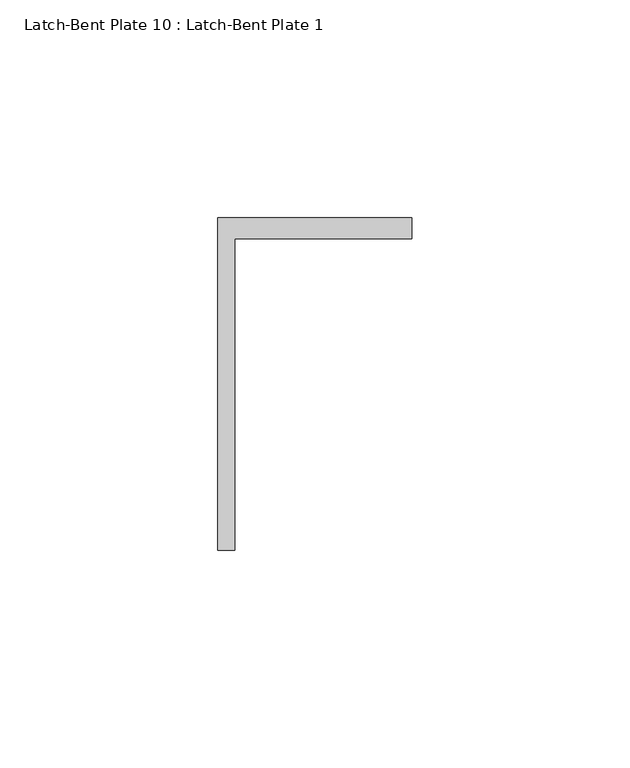
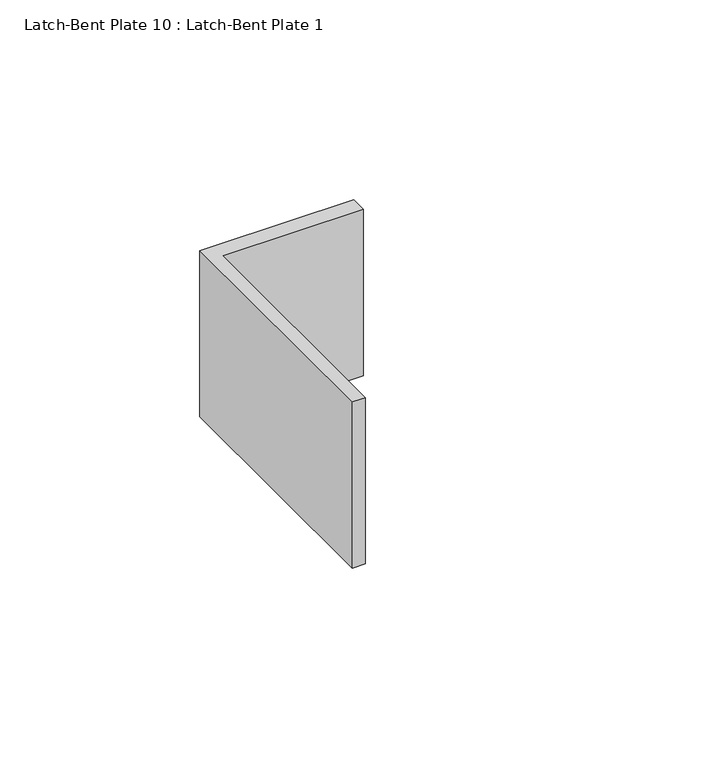
"""IFC4 building model written with IfcOpenShell, lengths in millimetres: proxy geometry, Latch-Bent Plate 10 : Latch-Bent Plate 1."""

import ifcopenshell
import ifcopenshell.guid

model = None  # the IFC model being written
_history = None  # IfcOwnerHistory: only IFC2X3 demands one
_inside = {}  # id of a spatial element -> (the spatial element, [elements in it])
_under = {}  # id of a project, library or spatial element -> (it, [spatial elements below it])
_declared = {}  # id of a project -> (the project, [libraries it declares])
_typed = {}  # id of a type object -> (the type object, [elements of that type])
_made_of = {}  # id of a material, layer set ... -> (it, [elements and type objects made of it])


def new_model(schema):
    """Start an empty IFC model of exactly this schema.

    Asked for "IFC4X3", IfcOpenShell would pick the latest addendum, in which some entities
    have other attributes; the version numbers below select the first issue.
    IFC2X3 requires an IfcOwnerHistory on every rooted entity: one is made here for all.
    """
    global model, _history
    if schema == "IFC4X3":
        model = ifcopenshell.file(schema_version=(4, 3, 0, 0))
    else:
        model = ifcopenshell.file(schema=schema)
    _inside.clear()
    _under.clear()
    _declared.clear()
    _typed.clear()
    _made_of.clear()
    _history = None
    if model.schema == "IFC2X3":
        org = make("IfcOrganization", Name="unknown")
        user = make(
            "IfcPersonAndOrganization",
            ThePerson=make("IfcPerson", FamilyName="unknown"),
            TheOrganization=org,
        )
        app = make(
            "IfcApplication",
            ApplicationDeveloper=org,
            Version="unknown",
            ApplicationFullName="unknown",
            ApplicationIdentifier="unknown",
        )
        _history = make(
            "IfcOwnerHistory",
            OwningUser=user,
            OwningApplication=app,
            ChangeAction="ADDED",
            CreationDate=0,
        )
    return model


def make(cls, **values):
    """One entity of the class cls with the attributes given. An attribute that is None is left unset."""
    return model.create_entity(
        cls, **{name: value for name, value in values.items() if value is not None}
    )


def rooted(cls, **values):
    """An entity with a GlobalId (a new one), such as an element, a storey or a relation."""
    return make(cls, GlobalId=ifcopenshell.guid.new(), OwnerHistory=_history, **values)


def si_unit(unit_type, name, prefix=None):
    """IfcSIUnit, for example si_unit("LENGTHUNIT", "METRE", prefix="MILLI")."""
    return make("IfcSIUnit", UnitType=unit_type, Prefix=prefix, Name=name)


def assignment(units):
    """IfcUnitAssignment: the units of a project."""
    return None if units is None else make("IfcUnitAssignment", Units=units)


def point(xyz):
    """IfcCartesianPoint."""
    return None if xyz is None else make("IfcCartesianPoint", Coordinates=xyz)


def direction(xyz):
    """IfcDirection."""
    return None if xyz is None else make("IfcDirection", DirectionRatios=xyz)


def frame(location, z_axis=None, x_axis=None):
    """IfcAxis2Placement3D, a coordinate frame: its origin and axes. An axis left out is left unset."""
    return make(
        "IfcAxis2Placement3D",
        Location=point(location),
        Axis=direction(z_axis),
        RefDirection=direction(x_axis),
    )


def origin():
    """The frame at (0, 0, 0) with its axes left unset."""
    return frame((0.0, 0.0, 0.0))


def place(relative_to, where):
    """IfcLocalPlacement: puts the frame where relative to a parent placement (None: the world)."""
    return make(
        "IfcLocalPlacement", PlacementRelTo=relative_to, RelativePlacement=where
    )


def context(
    kind, dimensions, precision=None, world=None, true_north=None, identifier=None
):
    """IfcGeometricRepresentationContext, for example the 3D "Model" context."""
    return make(
        "IfcGeometricRepresentationContext",
        ContextIdentifier=identifier,
        ContextType=kind,
        CoordinateSpaceDimension=dimensions,
        Precision=precision,
        WorldCoordinateSystem=world,
        TrueNorth=true_north,
    )


def project(units=None, contexts=None):
    """IfcProject with its units and contexts."""
    return rooted(
        "IfcProject",
        Name="project",
        RepresentationContexts=contexts,
        UnitsInContext=assignment(units),
    )


def spatial(cls, under=None, at=None, **own):
    """A site, building, storey or space (cls), placed at a placement, below another one or the project."""
    s = rooted(cls, ObjectPlacement=at, **own)
    if under is not None:
        _under.setdefault(under.id(), (under, []))[1].append(s)
    return s


def polyline(points):
    """IfcPolyline through the points."""
    return make("IfcPolyline", Points=[point(p) for p in points])


def outline(outer, holes=None, kind="AREA"):
    """IfcArbitraryClosedProfileDef: a profile drawn as a closed curve; with holes, ...WithVoids."""
    if holes is None:
        return make("IfcArbitraryClosedProfileDef", ProfileType=kind, OuterCurve=outer)
    return make(
        "IfcArbitraryProfileDefWithVoids",
        ProfileType=kind,
        OuterCurve=outer,
        InnerCurves=holes,
    )


def extrude(swept, where, along, depth):
    """IfcExtrudedAreaSolid: the profile swept, set in the frame where, extruded along a direction by depth."""
    return make(
        "IfcExtrudedAreaSolid",
        SweptArea=swept,
        Position=where,
        ExtrudedDirection=direction(along),
        Depth=depth,
    )


def shape(context_of_items, identifier, shape_type, items):
    """IfcShapeRepresentation: the items that make up one representation, for example the "Body"."""
    return make(
        "IfcShapeRepresentation",
        ContextOfItems=context_of_items,
        RepresentationIdentifier=identifier,
        RepresentationType=shape_type,
        Items=items,
    )


def source(mapping_origin, context_of_items, identifier, shape_type, items):
    """IfcRepresentationMap: a shape defined once, which mapped items show again and again."""
    return make(
        "IfcRepresentationMap",
        MappingOrigin=mapping_origin,
        MappedRepresentation=shape(context_of_items, identifier, shape_type, items),
    )


def transform(
    local_origin,
    x_axis=None,
    y_axis=None,
    z_axis=None,
    scale=None,
    scale2=None,
    scale3=None,
    uniform=True,
):
    """IfcCartesianTransformationOperator3D, or its non-uniform kind. x_axis, y_axis, z_axis: its Axis1, 2, 3."""
    if uniform:
        return make(
            "IfcCartesianTransformationOperator3D",
            Axis1=direction(x_axis),
            Axis2=direction(y_axis),
            LocalOrigin=point(local_origin),
            Scale=scale,
            Axis3=direction(z_axis),
        )
    return make(
        "IfcCartesianTransformationOperator3DnonUniform",
        Axis1=direction(x_axis),
        Axis2=direction(y_axis),
        LocalOrigin=point(local_origin),
        Scale=scale,
        Axis3=direction(z_axis),
        Scale2=scale2,
        Scale3=scale3,
    )


def mapped(mapping_source, mapping_target):
    """IfcMappedItem: shows the shape of a source again, moved by a transform."""
    return make(
        "IfcMappedItem", MappingSource=mapping_source, MappingTarget=mapping_target
    )


def made_of(thing, what):
    """Note that an element or type object is made of a material, layer set ...; save() writes the relation."""
    if what is not None:
        _made_of.setdefault(what.id(), (what, []))[1].append(thing)
    return thing


def element(
    cls,
    number,
    at=None,
    inside=None,
    cuts=None,
    type_object=None,
    material=None,
    context=None,
    identifier="Body",
    shape_type=None,
    held_by="IfcProductDefinitionShape",
    body=None,
    shapes=None,
    **own,
):
    """One element of the class cls, such as IfcWall. Its Tag is "e" and its number.

    at: its placement. inside: the storey or other place that contains it. cuts: it is an
    opening in that element (IfcRelVoidsElement). A single representation is given by context,
    identifier, shape_type and body (its items); several are given by shapes. held_by: the class
    of the entity that holds the representations. save() writes the other relations.
    """
    e = rooted(cls, Tag="e%d" % number, ObjectPlacement=at, **own)
    if body is not None:
        shapes = [shape(context, identifier, shape_type, body)]
    if shapes is not None:
        e.Representation = make(held_by, Representations=shapes)
    if inside is not None:
        _inside.setdefault(inside.id(), (inside, []))[1].append(e)
    if cuts is not None:
        rooted(
            "IfcRelVoidsElement", RelatingBuildingElement=cuts, RelatedOpeningElement=e
        )
    if type_object is not None:
        _typed.setdefault(type_object.id(), (type_object, []))[1].append(e)
    return made_of(e, material)


def aggregate(whole, parts):
    """IfcRelAggregates: a whole, such as a stair, and the parts it consists of."""
    return rooted("IfcRelAggregates", RelatingObject=whole, RelatedObjects=parts)


def save(model, path):
    """Write the relations noted so far, then the file.

    IfcRelAggregates (storeys below a building ...), IfcRelContainedInSpatialStructure (elements
    in a storey), IfcRelDefinesByType, IfcRelAssociatesMaterial and IfcRelDeclares: one each for
    every whole, place, type object, material and project.
    """
    for whole, parts in _under.values():
        aggregate(whole, parts)
    for where, things in _inside.values():
        rooted(
            "IfcRelContainedInSpatialStructure",
            RelatedElements=things,
            RelatingStructure=where,
        )
    for kind, things in _typed.values():
        rooted("IfcRelDefinesByType", RelatedObjects=things, RelatingType=kind)
    for what, things in _made_of.values():
        rooted("IfcRelAssociatesMaterial", RelatedObjects=things, RelatingMaterial=what)
    for by, libraries in _declared.values():
        rooted("IfcRelDeclares", RelatingContext=by, RelatedDefinitions=libraries)
    model.write(path)


def latch_bent_plate_10_latch_bent_plate_1_12525892(model_context):
    return source(origin(), model_context, "Body", "SweptSolid", [
        extrude(outline(polyline([(587327.0060739, -532883.8163841), (587366.6808739, -532883.8163841), (587366.6808739, -532888.5788841), (587326.1141748, -532888.5788841), (587326.1141748, -532960.0163841), (587322.2435739, -532960.0163841), (587322.2435739, -532883.8163841), (587327.0060739, -532883.8163841)])), frame((0.0, 0.0, 1041.4), z_axis=(0.0, 0.0, 1.0), x_axis=(1.0, 0.0, 0.0)), (0.0, 0.0, 1.0), 50.8),
    ])


if __name__ == "__main__":
    model = new_model("IFC4")
    model_context = context("Model", 3, world=origin())
    ifc_project = project(units=[si_unit("LENGTHUNIT", "METRE", prefix="MILLI")], contexts=[model_context])
    site = spatial("IfcSite", under=ifc_project)
    building = spatial("IfcBuilding", under=site)
    placement = place(None, origin())
    latch_bent_plate_10_latch_bent_plate_1_shape = latch_bent_plate_10_latch_bent_plate_1_12525892(model_context)
    element("IfcBuildingElementProxy", 1, Name="Latch-Bent Plate 10 : Latch-Bent Plate 1", ObjectType="Latch-Bent Plate 10 : Latch-Bent Plate 1", at=placement, inside=building, context=model_context, shape_type="MappedRepresentation", body=[
        mapped(latch_bent_plate_10_latch_bent_plate_1_shape, transform((0.0, 0.0, 0.0), x_axis=(1.0, 0.0, 0.0), y_axis=(0.0, 1.0, 0.0), z_axis=(0.0, 0.0, 1.0))),
    ])
    save(model, "model.ifc")

# Revit data of these elements
# Element 1 (IfcBuildingElementProxy, "Latch-Bent Plate 10 : Latch-Bent Plate 1")
#   Materials on its faces: "GALV. GATE LATCH"
# Materials
#   "GALV. GATE LATCH": class "Metal", colour RGB 189 187 185, transparency 0, Description = "Carbon steel", Cost = 0
